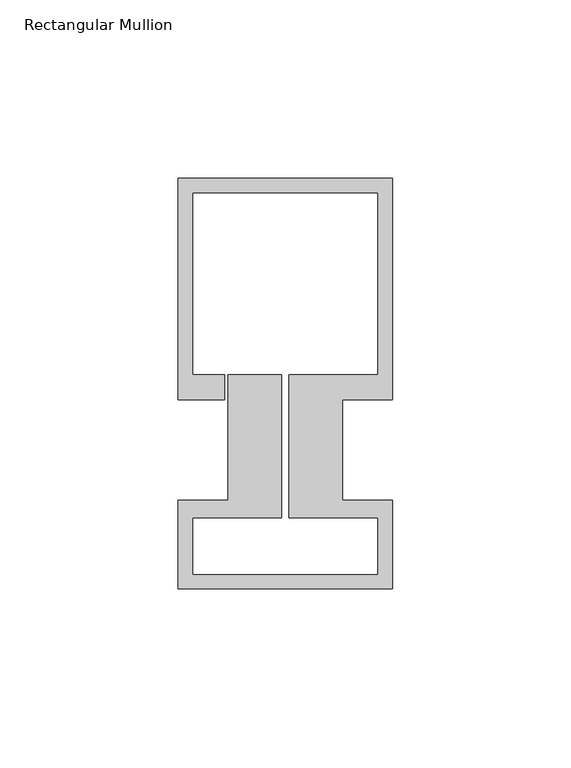
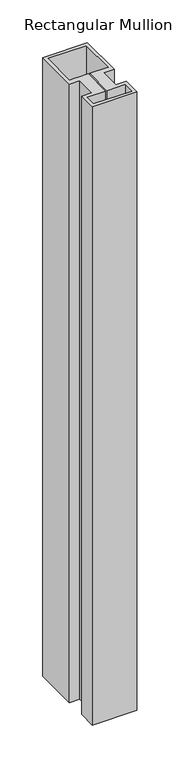
"""IFC4 building model written with IfcOpenShell, lengths in millimetres: member geometry, Rectangular Mullion : Schueco_FWS-60-HI_Tran_CovCap-20mm_Tran-55mm."""

from ifc_helpers import new_model, si_unit, frame, origin, place, context, project, spatial, polyline, outline, extrude, source, transform, mapped, element, save


def rectangular_mullion_50bdc20f(model_context):
    return source(origin(), model_context, "Body", "SweptSolid", [
        extrude(outline(polyline([(0.0, 90.0), (0.0, 28.0), (-14.0, 28.0), (-14.0, -0.1), (0.0, -0.1), (0.0, -25.0), (-60.0, -25.0), (-60.0, -0.1), (-46.0, -0.1), (-46.0, 35.0), (-31.0, 35.0), (-31.0, -5.0), (-56.0, -5.0), (-56.0, -21.0), (-4.0, -21.0), (-4.0, -5.0), (-29.0, -5.0), (-29.0, 35.0), (-4.0, 35.0), (-4.0, 86.0), (-56.0, 86.0), (-56.0, 35.0), (-47.0, 35.0), (-47.0, 28.0), (-60.0, 28.0), (-60.0, 90.0), (0.0, 90.0)])), frame((0.0, 0.0, -880.0), z_axis=(0.0, 0.0, 1.0), x_axis=(1.0, 0.0, 0.0)), (0.0, 0.0, 1.0), 880.0),
    ])


if __name__ == "__main__":
    model = new_model("IFC4")
    model_context = context("Model", 3, world=origin())
    ifc_project = project(units=[si_unit("LENGTHUNIT", "METRE", prefix="MILLI")], contexts=[model_context])
    site = spatial("IfcSite", under=ifc_project)
    building = spatial("IfcBuilding", under=site)
    placement = place(None, origin())
    rectangular_mullion_shape = rectangular_mullion_50bdc20f(model_context)
    element("IfcMember", 1, ObjectType="Rectangular Mullion : Schueco_FWS-60-HI_Tran_CovCap-20mm_Tran-55mm", at=placement, inside=building, context=model_context, shape_type="MappedRepresentation", body=[
        mapped(rectangular_mullion_shape, transform((0.0, 0.0, 0.0), x_axis=(1.0, 0.0, 0.0), y_axis=(0.0, 1.0, 0.0), z_axis=(0.0, 0.0, 1.0))),
    ])
    save(model, "model.ifc")

# Revit data of these elements
# Type "Rectangular Mullion : Schueco_FWS-60-HI_Tran_CovCap-20mm_Tran-55mm"
#   Model = "FWS 60.HI"
#   Manufacturer = "Schueco International KG"
#   Type Comments = "Transom"
#   Schueco thermal insulation standard = "Highly thermally insulated"
#   Burglar resistance = "RC 3"
#   Thermal insulation = "to 0.90 W/(m²K)"
#   built-in parameter 1007322 = 0.377297 (stored number, unit not read)
#   built-in parameter 1007321 = 0.0524934 (stored number, unit not read)
#   built-in parameter 1007320 = 0.0524934 (stored number, unit not read)
# Element 1 (IfcMember, "Rectangular Mullion : Schueco_FWS-60-HI_Tran_CovCap-20mm_Tran-55mm")
#   Materials on its faces: "Alu"
# Materials
#   "Alu": class "Glas", colour RGB 140 140 140, transparency 0
